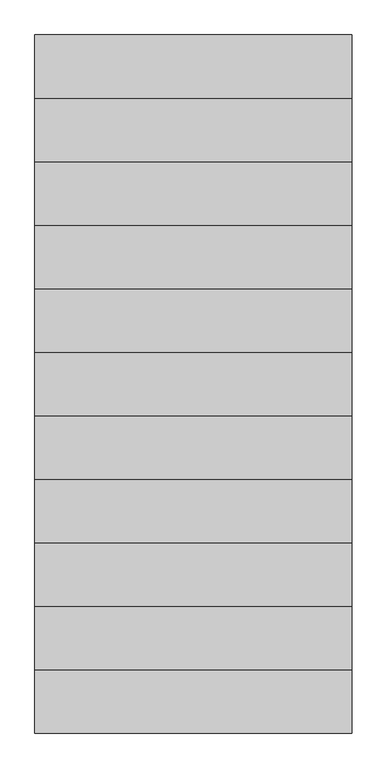
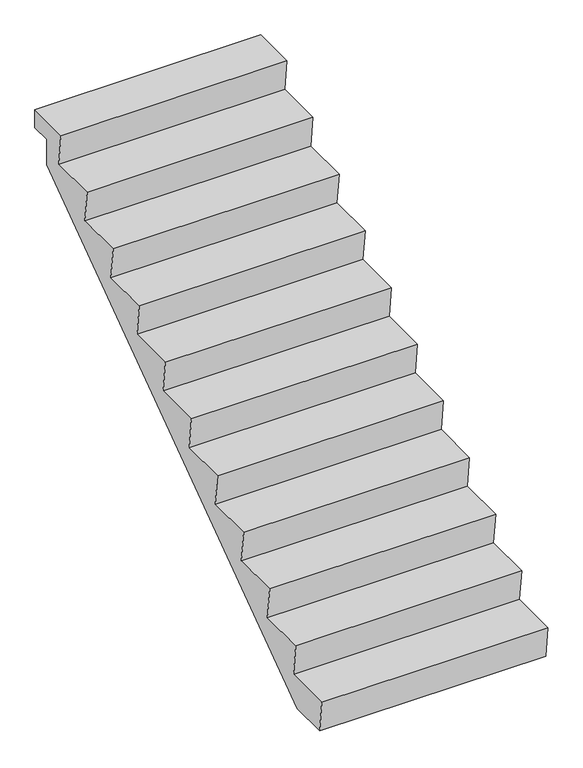
"""IFC4 building model written with IfcOpenShell, lengths in millimetres: proxy geometry, NLRS_24_GM_LB_rechte steektrap prefab-AV_gen_rsf : prefab trap_gen__aant=11 b=1200 a=220 o=172.7 zonder bomen onder geen oplegnok."""

from ifc_helpers import new_model, si_unit, frame, origin, place, context, project, spatial, polyline, outline, extrude, source, transform, mapped, element, save


def generic_models_0bdb91d7(model_context):
    return source(origin(), model_context, "Body", "SweptSolid", [
        extrude(outline(polyline([(2400.0, 1900.0), (2640.0, 1900.0), (2640.0, 1800.0), (2530.0, 1800.0), (2530.0, 1658.5925892), (225.4292445, 0.0), (20.0, 0.0), (0.0, 172.7272727), (260.0, 172.7272727), (240.0, 345.4545455), (500.0, 345.4545455), (480.0, 518.1818182), (740.0, 518.1818182), (720.0, 690.9090909), (980.0, 690.9090909), (960.0, 863.6363636), (1220.0, 863.6363636), (1200.0, 1036.3636364), (1460.0, 1036.3636364), (1440.0, 1209.0909091), (1700.0, 1209.0909091), (1680.0, 1381.8181818), (1940.0, 1381.8181818), (1920.0, 1554.5454545), (2180.0, 1554.5454545), (2160.0, 1727.2727273), (2420.0, 1727.2727273), (2400.0, 1900.0)])), frame((-600.0, 0.0, 0.0), z_axis=(1.0, 0.0, 0.0), x_axis=(0.0, 1.0, 0.0)), (0.0, 0.0, 1.0), 1200.0),
    ])


if __name__ == "__main__":
    model = new_model("IFC4")
    model_context = context("Model", 3, world=origin())
    ifc_project = project(units=[si_unit("LENGTHUNIT", "METRE", prefix="MILLI")], contexts=[model_context])
    site = spatial("IfcSite", under=ifc_project)
    building = spatial("IfcBuilding", under=site)
    placement = place(None, origin())
    generic_models_shape = generic_models_0bdb91d7(model_context)
    element("IfcBuildingElementProxy", 1, Name="NLRS_24_GM_LB_rechte steektrap prefab-AV_gen_rsf : prefab trap_gen__aant=11 b=1200 a=220 o=172.7 zonder bomen onder geen oplegnok", ObjectType="NLRS_24_GM_LB_rechte steektrap prefab-AV_gen_rsf : prefab trap_gen__aant=11 b=1200 a=220 o=172.7 zonder bomen onder geen oplegnok", at=placement, inside=building, context=model_context, shape_type="MappedRepresentation", body=[
        mapped(generic_models_shape, transform((0.0, 0.0, 0.0), x_axis=(1.0, 0.0, 0.0), y_axis=(0.0, 1.0, 0.0), z_axis=(0.0, 0.0, 1.0))),
    ])
    save(model, "model.ifc")

# Revit data of these elements
# Type "NLRS_24_GM_LB_rechte steektrap prefab-AV_gen_rsf : prefab trap_gen__aant=11 b=1200 a=220 o=172.7 zonder bomen onder geen oplegnok"
#   Export Type to IFC As = "IfcStair"
#   Type IfcGUID = "2CEqVLPNH8KRN7ghwV3aZy"
#   Type Comments = " "
#   Model = " "
#   Manufacturer = " "
#   Keynote = " "
#   Description = "rechte steektrap prefab\r\naant=11 b=1200 a=220 o=181,8\r\nzonder bomen"
#   Assembly Code = "24.11"
#   Aantrede onder = 240 mm
#   Width = 1200 mm
#   Wel diepte = 20 mm
#   Trapboom breedte = 0 mm
#   Thickness = 120 mm
#   Optrede onderste trede = 220 mm
#   NLRS_C_lengte = 2400 mm
#   Length = 2880 mm
#   Hoogte oplegnok onder = 100 mm
#   Hoogte oplegnok boven = 100 mm
#   Height = 1900 mm
#   Breedte oplegnok boven = 110 mm
#   BottomCalc = 220 mm
#   Actual Tread Depth = 240 mm
#   Actual Riser Height = 172.727 mm
#   Actual Number of Tread = 10
#   Actual Number of Risers = 11
#   Aantrede boven = 240 mm
#   Aantal treden max dertig = 11
#   Trapboom = no
#   Oplegnok onder = no
#   NLRS_C_materiaal = NLRS_f2_beton prefab_gen_rsf
#   Default Elevation = 0
# Element 1 (IfcBuildingElementProxy, "NLRS_24_GM_LB_rechte steektrap prefab-AV_gen_rsf : prefab trap_gen__aant=11 b=1200 a=220 o=172.7 zonder bomen onder geen oplegnok")
#   Materials on its faces: "NLRS_f2_beton prefab_gen_rsf"
# Materials
#   "NLRS_f2_beton prefab_gen_rsf": class "F - Niet gebakken kunststeen", colour RGB 129 133 118, transparency 0, Keynote = "f2", Manufacturer = "Revit Standards Foundation", URL = "www.revitstandards.org", Description = "beton prefab", Cost = 0
